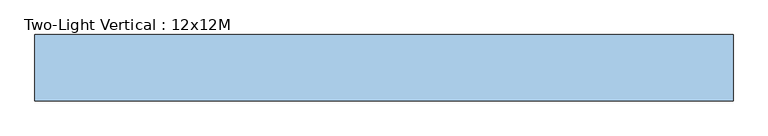
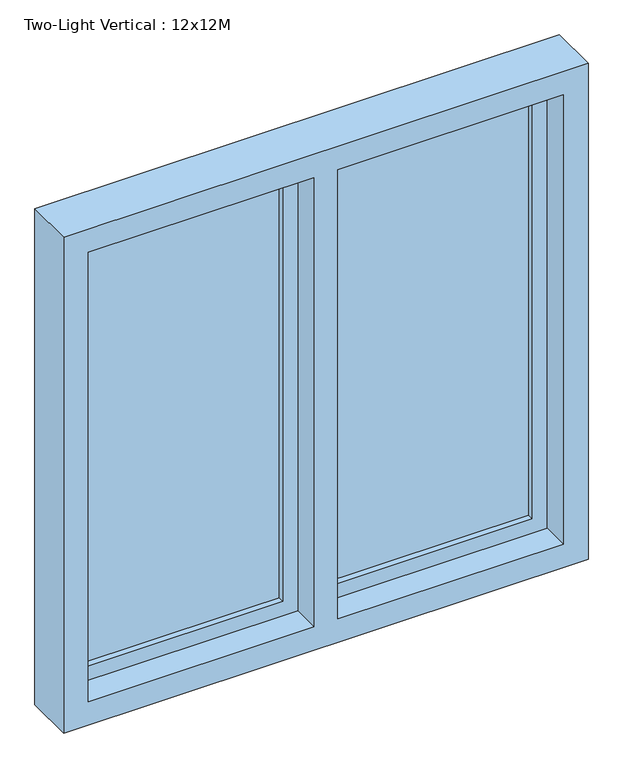
"""IFC4 building model written with IfcOpenShell, lengths in millimetres: window geometry, Two-Light Vertical : 12x12M."""

import ifcopenshell
import ifcopenshell.guid

model = None  # the IFC model being written
_history = None  # IfcOwnerHistory: only IFC2X3 demands one
_inside = {}  # id of a spatial element -> (the spatial element, [elements in it])
_under = {}  # id of a project, library or spatial element -> (it, [spatial elements below it])
_declared = {}  # id of a project -> (the project, [libraries it declares])
_typed = {}  # id of a type object -> (the type object, [elements of that type])
_made_of = {}  # id of a material, layer set ... -> (it, [elements and type objects made of it])


def new_model(schema):
    """Start an empty IFC model of exactly this schema.

    Asked for "IFC4X3", IfcOpenShell would pick the latest addendum, in which some entities
    have other attributes; the version numbers below select the first issue.
    IFC2X3 requires an IfcOwnerHistory on every rooted entity: one is made here for all.
    """
    global model, _history
    if schema == "IFC4X3":
        model = ifcopenshell.file(schema_version=(4, 3, 0, 0))
    else:
        model = ifcopenshell.file(schema=schema)
    _inside.clear()
    _under.clear()
    _declared.clear()
    _typed.clear()
    _made_of.clear()
    _history = None
    if model.schema == "IFC2X3":
        org = make("IfcOrganization", Name="unknown")
        user = make(
            "IfcPersonAndOrganization",
            ThePerson=make("IfcPerson", FamilyName="unknown"),
            TheOrganization=org,
        )
        app = make(
            "IfcApplication",
            ApplicationDeveloper=org,
            Version="unknown",
            ApplicationFullName="unknown",
            ApplicationIdentifier="unknown",
        )
        _history = make(
            "IfcOwnerHistory",
            OwningUser=user,
            OwningApplication=app,
            ChangeAction="ADDED",
            CreationDate=0,
        )
    return model


def make(cls, **values):
    """One entity of the class cls with the attributes given. An attribute that is None is left unset."""
    return model.create_entity(
        cls, **{name: value for name, value in values.items() if value is not None}
    )


def rooted(cls, **values):
    """An entity with a GlobalId (a new one), such as an element, a storey or a relation."""
    return make(cls, GlobalId=ifcopenshell.guid.new(), OwnerHistory=_history, **values)


def si_unit(unit_type, name, prefix=None):
    """IfcSIUnit, for example si_unit("LENGTHUNIT", "METRE", prefix="MILLI")."""
    return make("IfcSIUnit", UnitType=unit_type, Prefix=prefix, Name=name)


def assignment(units):
    """IfcUnitAssignment: the units of a project."""
    return None if units is None else make("IfcUnitAssignment", Units=units)


def point(xyz):
    """IfcCartesianPoint."""
    return None if xyz is None else make("IfcCartesianPoint", Coordinates=xyz)


def direction(xyz):
    """IfcDirection."""
    return None if xyz is None else make("IfcDirection", DirectionRatios=xyz)


def frame(location, z_axis=None, x_axis=None):
    """IfcAxis2Placement3D, a coordinate frame: its origin and axes. An axis left out is left unset."""
    return make(
        "IfcAxis2Placement3D",
        Location=point(location),
        Axis=direction(z_axis),
        RefDirection=direction(x_axis),
    )


def origin():
    """The frame at (0, 0, 0) with its axes left unset."""
    return frame((0.0, 0.0, 0.0))


def place(relative_to, where):
    """IfcLocalPlacement: puts the frame where relative to a parent placement (None: the world)."""
    return make(
        "IfcLocalPlacement", PlacementRelTo=relative_to, RelativePlacement=where
    )


def context(
    kind, dimensions, precision=None, world=None, true_north=None, identifier=None
):
    """IfcGeometricRepresentationContext, for example the 3D "Model" context."""
    return make(
        "IfcGeometricRepresentationContext",
        ContextIdentifier=identifier,
        ContextType=kind,
        CoordinateSpaceDimension=dimensions,
        Precision=precision,
        WorldCoordinateSystem=world,
        TrueNorth=true_north,
    )


def project(units=None, contexts=None):
    """IfcProject with its units and contexts."""
    return rooted(
        "IfcProject",
        Name="project",
        RepresentationContexts=contexts,
        UnitsInContext=assignment(units),
    )


def spatial(cls, under=None, at=None, **own):
    """A site, building, storey or space (cls), placed at a placement, below another one or the project."""
    s = rooted(cls, ObjectPlacement=at, **own)
    if under is not None:
        _under.setdefault(under.id(), (under, []))[1].append(s)
    return s


def polyline(points):
    """IfcPolyline through the points."""
    return make("IfcPolyline", Points=[point(p) for p in points])


def outline(outer, holes=None, kind="AREA"):
    """IfcArbitraryClosedProfileDef: a profile drawn as a closed curve; with holes, ...WithVoids."""
    if holes is None:
        return make("IfcArbitraryClosedProfileDef", ProfileType=kind, OuterCurve=outer)
    return make(
        "IfcArbitraryProfileDefWithVoids",
        ProfileType=kind,
        OuterCurve=outer,
        InnerCurves=holes,
    )


def extrude(swept, where, along, depth):
    """IfcExtrudedAreaSolid: the profile swept, set in the frame where, extruded along a direction by depth."""
    return make(
        "IfcExtrudedAreaSolid",
        SweptArea=swept,
        Position=where,
        ExtrudedDirection=direction(along),
        Depth=depth,
    )


def faces_of(points, faces, orient=None, outer=None):
    """IfcFace entities. A face is a list of loops; a loop is a list of indices into points, from 0.

    orient and outer hold one flag for each loop. By default every Orientation is true, the
    first loop of a face is its IfcFaceOuterBound and the others are IfcFaceBound.
    """
    made = []
    for i, loops in enumerate(faces):
        bounds = []
        for j, loop in enumerate(loops):
            is_outer = j == 0 if outer is None else outer[i][j]
            bounds.append(
                make(
                    "IfcFaceOuterBound" if is_outer else "IfcFaceBound",
                    Bound=make("IfcPolyLoop", Polygon=[points[k] for k in loop]),
                    Orientation=True if orient is None else orient[i][j],
                )
            )
        made.append(make("IfcFace", Bounds=bounds))
    return made


def faceted_brep(points, faces, orient=None, outer=None, voids=None):
    """IfcFacetedBrep: a solid bounded by flat faces; with voids (closed shells), ...WithVoids."""
    shared = [point(p) for p in points]
    hull = make("IfcClosedShell", CfsFaces=faces_of(shared, faces, orient, outer))
    if voids is None:
        return make("IfcFacetedBrep", Outer=hull)
    return make(
        "IfcFacetedBrepWithVoids",
        Outer=hull,
        Voids=[
            make(cls, CfsFaces=faces_of(shared, fs, o, b)) for cls, fs, o, b in voids
        ],
    )


def shape(context_of_items, identifier, shape_type, items):
    """IfcShapeRepresentation: the items that make up one representation, for example the "Body"."""
    return make(
        "IfcShapeRepresentation",
        ContextOfItems=context_of_items,
        RepresentationIdentifier=identifier,
        RepresentationType=shape_type,
        Items=items,
    )


def source(mapping_origin, context_of_items, identifier, shape_type, items):
    """IfcRepresentationMap: a shape defined once, which mapped items show again and again."""
    return make(
        "IfcRepresentationMap",
        MappingOrigin=mapping_origin,
        MappedRepresentation=shape(context_of_items, identifier, shape_type, items),
    )


def transform(
    local_origin,
    x_axis=None,
    y_axis=None,
    z_axis=None,
    scale=None,
    scale2=None,
    scale3=None,
    uniform=True,
):
    """IfcCartesianTransformationOperator3D, or its non-uniform kind. x_axis, y_axis, z_axis: its Axis1, 2, 3."""
    if uniform:
        return make(
            "IfcCartesianTransformationOperator3D",
            Axis1=direction(x_axis),
            Axis2=direction(y_axis),
            LocalOrigin=point(local_origin),
            Scale=scale,
            Axis3=direction(z_axis),
        )
    return make(
        "IfcCartesianTransformationOperator3DnonUniform",
        Axis1=direction(x_axis),
        Axis2=direction(y_axis),
        LocalOrigin=point(local_origin),
        Scale=scale,
        Axis3=direction(z_axis),
        Scale2=scale2,
        Scale3=scale3,
    )


def mapped(mapping_source, mapping_target):
    """IfcMappedItem: shows the shape of a source again, moved by a transform."""
    return make(
        "IfcMappedItem", MappingSource=mapping_source, MappingTarget=mapping_target
    )


def made_of(thing, what):
    """Note that an element or type object is made of a material, layer set ...; save() writes the relation."""
    if what is not None:
        _made_of.setdefault(what.id(), (what, []))[1].append(thing)
    return thing


def element(
    cls,
    number,
    at=None,
    inside=None,
    cuts=None,
    type_object=None,
    material=None,
    context=None,
    identifier="Body",
    shape_type=None,
    held_by="IfcProductDefinitionShape",
    body=None,
    shapes=None,
    **own,
):
    """One element of the class cls, such as IfcWall. Its Tag is "e" and its number.

    at: its placement. inside: the storey or other place that contains it. cuts: it is an
    opening in that element (IfcRelVoidsElement). A single representation is given by context,
    identifier, shape_type and body (its items); several are given by shapes. held_by: the class
    of the entity that holds the representations. save() writes the other relations.
    """
    e = rooted(cls, Tag="e%d" % number, ObjectPlacement=at, **own)
    if body is not None:
        shapes = [shape(context, identifier, shape_type, body)]
    if shapes is not None:
        e.Representation = make(held_by, Representations=shapes)
    if inside is not None:
        _inside.setdefault(inside.id(), (inside, []))[1].append(e)
    if cuts is not None:
        rooted(
            "IfcRelVoidsElement", RelatingBuildingElement=cuts, RelatedOpeningElement=e
        )
    if type_object is not None:
        _typed.setdefault(type_object.id(), (type_object, []))[1].append(e)
    return made_of(e, material)


def aggregate(whole, parts):
    """IfcRelAggregates: a whole, such as a stair, and the parts it consists of."""
    return rooted("IfcRelAggregates", RelatingObject=whole, RelatedObjects=parts)


def save(model, path):
    """Write the relations noted so far, then the file.

    IfcRelAggregates (storeys below a building ...), IfcRelContainedInSpatialStructure (elements
    in a storey), IfcRelDefinesByType, IfcRelAssociatesMaterial and IfcRelDeclares: one each for
    every whole, place, type object, material and project.
    """
    for whole, parts in _under.values():
        aggregate(whole, parts)
    for where, things in _inside.values():
        rooted(
            "IfcRelContainedInSpatialStructure",
            RelatedElements=things,
            RelatingStructure=where,
        )
    for kind, things in _typed.values():
        rooted("IfcRelDefinesByType", RelatedObjects=things, RelatingType=kind)
    for what, things in _made_of.values():
        rooted("IfcRelAssociatesMaterial", RelatedObjects=things, RelatingMaterial=what)
    for by, libraries in _declared.values():
        rooted("IfcRelDeclares", RelatingContext=by, RelatedDefinitions=libraries)
    model.write(path)


def two_light_vertical_12x12m_7e3a313f(model_context):
    return source(origin(), model_context, "Body", "SolidModel", [
        extrude(outline(polyline([(1970.0, -624.0), (842.0, -624.0), (842.0, -72.5), (1970.0, -72.5), (1970.0, -624.0)]), holes=[polyline([(1920.0, -122.5), (892.0, -122.5), (892.0, -574.0), (1920.0, -574.0), (1920.0, -122.5)])]), frame((0.0, 134.0, 0.0), z_axis=(0.0, 1.0, 0.0), x_axis=(0.0, 0.0, 1.0)), (0.0, 0.0, 1.0), 50.0),
        extrude(outline(polyline([(1970.0, -47.5), (842.0, -47.5), (842.0, 504.0), (1970.0, 504.0), (1970.0, -47.5)]), holes=[polyline([(1920.0, 454.0), (892.0, 454.0), (892.0, 2.5), (1920.0, 2.5), (1920.0, 454.0)])]), frame((0.0, 134.0, 0.0), z_axis=(0.0, 1.0, 0.0), x_axis=(0.0, 0.0, 1.0)), (0.0, 0.0, 1.0), 50.0),
        faceted_brep([(-666.0, 184.0, 800.0), (546.0, 184.0, 800.0), (546.0, 69.0, 800.0), (-666.0, 69.0, 800.0), (546.0, 184.0, 2012.0), (546.0, 69.0, 2012.0), (-666.0, 184.0, 2012.0), (504.0, 184.0, 842.0), (504.0, 184.0, 1970.0), (-47.5, 184.0, 1970.0), (-47.5, 184.0, 842.0), (-624.0, 184.0, 842.0), (-72.5, 184.0, 842.0), (-72.5, 184.0, 1970.0), (-624.0, 184.0, 1970.0), (-666.0, 69.0, 2012.0), (489.0, 69.0, 1955.0), (489.0, 69.0, 857.0), (-32.5, 69.0, 857.0), (-32.5, 69.0, 1955.0), (-609.0, 69.0, 1955.0), (-87.5, 69.0, 1955.0), (-87.5, 69.0, 857.0), (-609.0, 69.0, 857.0), (489.0, 134.0, 857.0), (-32.5, 134.0, 857.0), (-609.0, 134.0, 857.0), (-87.5, 134.0, 857.0), (489.0, 134.0, 1955.0), (504.0, 134.0, 1970.0), (504.0, 134.0, 842.0), (-47.5, 134.0, 842.0), (-47.5, 134.0, 1970.0), (-32.5, 134.0, 1955.0), (-624.0, 134.0, 842.0), (-624.0, 134.0, 1970.0), (-72.5, 134.0, 1970.0), (-72.5, 134.0, 842.0), (-609.0, 134.0, 1955.0), (-87.5, 134.0, 1955.0)], [[[0, 1, 2, 3]], [[2, 1, 4, 5]], [[4, 1, 0, 6], [7, 8, 9, 10], [11, 12, 13, 14]], [[2, 5, 15, 3], [16, 17, 18, 19], [20, 21, 22, 23]], [[17, 24, 25, 18]], [[26, 23, 22, 27]], [[24, 17, 16, 28]], [[29, 30, 31, 32], [24, 28, 33, 25]], [[34, 35, 36, 37], [38, 26, 27, 39]], [[31, 30, 7, 10]], [[11, 34, 37, 12]], [[7, 30, 29, 8]], [[15, 6, 0, 3]], [[38, 20, 23, 26]], [[14, 35, 34, 11]], [[10, 9, 32, 31]], [[19, 18, 25, 33]], [[22, 21, 39, 27]], [[13, 12, 37, 36]], [[15, 5, 4, 6]], [[28, 16, 19, 33]], [[20, 38, 39, 21]], [[8, 29, 32, 9]], [[36, 35, 14, 13]]]),
        extrude(outline(polyline([(-574.0, 170.0), (-122.5, 170.0), (-122.5, 148.0), (-574.0, 148.0), (-574.0, 170.0)])), frame((0.0, 0.0, 892.0), z_axis=(0.0, 0.0, 1.0), x_axis=(1.0, 0.0, 0.0)), (0.0, 0.0, 1.0), 1028.0),
        extrude(outline(polyline([(2.5, 170.0), (454.0, 170.0), (454.0, 148.0), (2.5, 148.0), (2.5, 170.0)])), frame((0.0, 0.0, 892.0), z_axis=(0.0, 0.0, 1.0), x_axis=(1.0, 0.0, 0.0)), (0.0, 0.0, 1.0), 1028.0),
    ])


if __name__ == "__main__":
    model = new_model("IFC4")
    model_context = context("Model", 3, world=origin())
    ifc_project = project(units=[si_unit("LENGTHUNIT", "METRE", prefix="MILLI")], contexts=[model_context])
    site = spatial("IfcSite", under=ifc_project)
    building = spatial("IfcBuilding", under=site)
    placement = place(None, origin())
    two_light_vertical_12x12m_shape = two_light_vertical_12x12m_7e3a313f(model_context)
    element("IfcWindow", 1, ObjectType="Two-Light Vertical : 12x12M", at=placement, inside=building, context=model_context, shape_type="MappedRepresentation", body=[
        mapped(two_light_vertical_12x12m_shape, transform((0.0, 0.0, 0.0), x_axis=(1.0, 0.0, 0.0), y_axis=(0.0, 1.0, 0.0), z_axis=(0.0, 0.0, 1.0))),
    ])
    save(model, "model.ifc")

# Revit data of these elements
# Type "Two-Light Vertical : 12x12M"
#   Type Mark = "52"
#   Creator Organization [instance default] = "© Danish Educational Content"
#   Creator Name [instance default] = "© Erik Falck Jørgensen"
#   Creator Build [instance default] = "2017.0801.0"
#   Analytic Construction = "<None>"
#   length#5 = -36 mm
#   length#4 = -14 mm
#   length#3 = 120 mm
#   length#2 = 57 mm
#   length#1 = 0 mm
#   Seal Width = 12 mm
#   Rough Width = 1212 mm
#   Rough Height = 1212 mm
#   Rabbet Width = 15 mm
#   Rebate Depth = 50 mm
#   Transom Width = 55 mm
#   Rabbet Depth = 50 mm
#   Height = 1188 mm
#   Glass Thickness = 22 mm
#   Frame Width = 50 mm
#   Frame Depth = 50 mm
#   Exterior Direction [instance default] = 0.00°
#   Case Depth = 115 mm
#   Case Width = 45 mm
#   Default Sill Height = 800 mm
#   Width = 1188 mm
#   Sealing = no
#   Hinging = yes
#   Wall Closure = 1
#   Above Cutplane [instance default] = no
#   Glass = none
#   Case/Transom = none
#   Frame/Mullion = none
#   Assembly Code = ""
# Element 1 (IfcWindow, "Two-Light Vertical : 12x12M")
#   Materials on its faces: "Default Frame/Mullion (Interior/Exterior)", "Glass"
# Materials
#   "Default Frame/Mullion (Interior/Exterior)": class "Generic", colour RGB 205 205 205, transparency 0, Description = "Udefineret karm/ramme materiale", Cost = 0
#   "Glass": class "Glass", colour RGB 180 200 255, transparency 0.75, Description = "Generisk glas", Cost = 0
